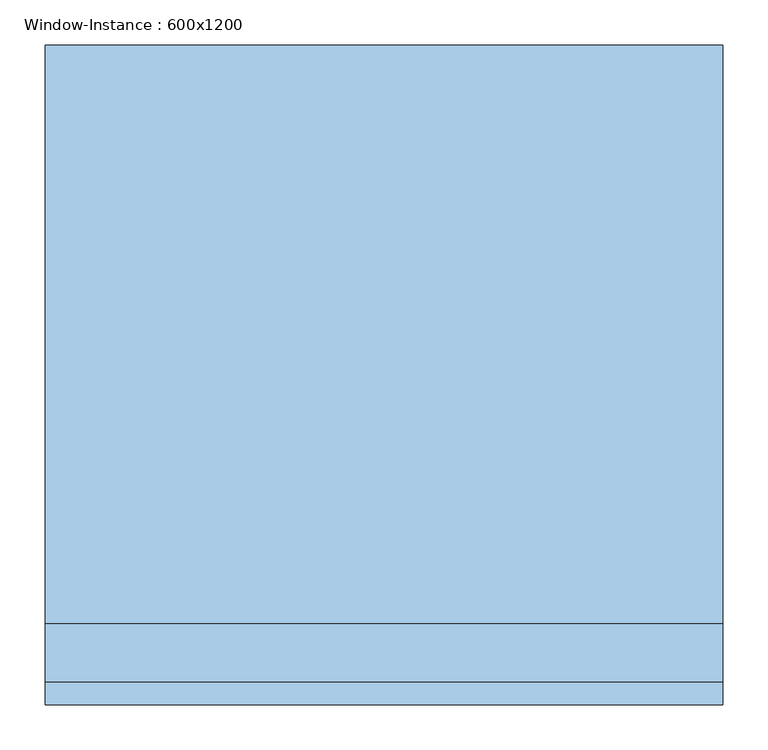
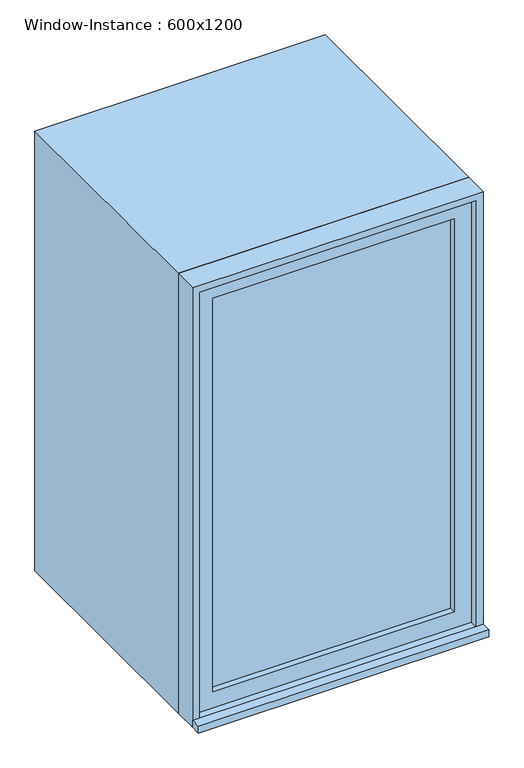
"""IFC4 building model written with IfcOpenShell, lengths in millimetres: window geometry, Window-Instance : 600x1200."""

from ifc_helpers import new_model, si_unit, frame, origin, place, context, project, spatial, polyline, outline, extrude, source, transform, mapped, element, save


def window_instance_600x1200_c4429aef(model_context):
    return source(origin(), model_context, "Body", "SweptSolid", [
        extrude(outline(polyline([(-413.1, -377.9), (-413.1, -352.5), (336.9, -352.5), (336.9, -377.9), (-413.1, -377.9)])), frame((0.0, 0.0, 900.0), z_axis=(0.0, 0.0, 1.0), x_axis=(1.0, 0.0, 0.0)), (0.0, 0.0, 1.0), 19.05),
        extrude(outline(polyline([(273.4, -303.925), (273.4, -316.625), (-349.6, -316.625), (-349.6, -303.925), (273.4, -303.925)])), frame((0.0, 0.0, 963.5), z_axis=(0.0, 0.0, 1.0), x_axis=(1.0, 0.0, 0.0)), (0.0, 0.0, 1.0), 1073.0),
        extrude(outline(polyline([(2080.95, -394.05), (919.05, -394.05), (919.05, 317.85), (2080.95, 317.85), (2080.95, -394.05)]), holes=[polyline([(2036.5, -349.6), (2036.5, 273.4), (963.5, 273.4), (963.5, -349.6), (2036.5, -349.6)])]), frame((0.0, -332.5, 0.0), z_axis=(0.0, 1.0, 0.0), x_axis=(0.0, 0.0, 1.0)), (0.0, 0.0, 1.0), 44.45),
        extrude(outline(polyline([(2100.0, -413.1), (900.0, -413.1), (900.0, 336.9), (2100.0, 336.9), (2100.0, -413.1)]), holes=[polyline([(2068.25, -381.35), (2068.25, 305.15), (931.75, 305.15), (931.75, -381.35), (2068.25, -381.35)])]), frame((0.0, -288.05, 0.0), z_axis=(0.0, 1.0, 0.0), x_axis=(0.0, 0.0, 1.0)), (0.0, 0.0, 1.0), 640.55),
        extrude(outline(polyline([(2100.0, 336.9), (2100.0, -413.1), (900.0, -413.1), (900.0, 336.9), (2100.0, 336.9)]), holes=[polyline([(2080.95, 317.85), (919.05, 317.85), (919.05, -394.05), (2080.95, -394.05), (2080.95, 317.85)])]), frame((0.0, -352.5, 0.0), z_axis=(0.0, 1.0, 0.0), x_axis=(0.0, 0.0, 1.0)), (0.0, 0.0, 1.0), 64.45),
    ])


if __name__ == "__main__":
    model = new_model("IFC4")
    model_context = context("Model", 3, world=origin())
    ifc_project = project(units=[si_unit("LENGTHUNIT", "METRE", prefix="MILLI")], contexts=[model_context])
    site = spatial("IfcSite", under=ifc_project)
    building = spatial("IfcBuilding", under=site)
    placement = place(None, origin())
    window_instance_600x1200_shape = window_instance_600x1200_c4429aef(model_context)
    element("IfcWindow", 1, ObjectType="Window-Instance : 600x1200", at=placement, inside=building, context=model_context, shape_type="MappedRepresentation", body=[
        mapped(window_instance_600x1200_shape, transform((0.0, 0.0, 0.0), x_axis=(1.0, 0.0, 0.0), y_axis=(0.0, 1.0, 0.0), z_axis=(0.0, 0.0, 1.0))),
    ])
    save(model, "model.ifc")

# Revit data of these elements
# Type "Window-Instance : 600x1200"
#   Type Mark = "7"
#   Construction Type Id = "GSP4R"
#   Assembly Code = "B2020100"
#   Analytic Construction = "1/8 in Pilkington single glazing"
#   Visual Light Transmittance = 0.9
#   Thermal Resistance (R) = 0.149095 (m²·K)/W
#   Solar Heat Gain Coefficient = 0.86
#   Heat Transfer Coefficient (U) = 6.70716 W/(m²·K)
#   Height [instance default] = 1200 mm
#   Default Sill Height = 900 mm
#   Width [instance default] = 600 mm
#   Window Inset = 20 mm
#   Glass Pane Material = WW-EC-GL-Storefront
#   Sash Material = WW-EC-RGB-White
#   Wall Closure = (empty or 0)
# Element 1 (IfcWindow, "Window-Instance : 600x1200")
#   Width = 750 mm
#   Materials on its faces: "WW-EC-RGB-White", "WW-EC-GL-Storefront"
# Materials
#   "WW-EC-GL-Storefront": class "Glass", colour RGB 236 240 239, transparency 0.85, Description = "Storefront Glass", Cost = 0
#   "WW-EC-RGB-White": class "Generic", colour RGB 255 255 255, transparency 0, Comments = "If region requests off-white, swith asset color to RGB 231-228-220", Description = "Generic Color", Cost = 0
